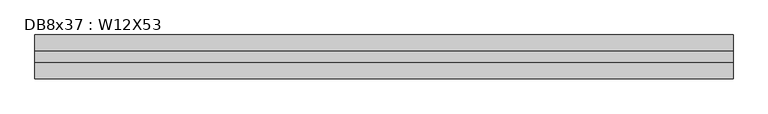
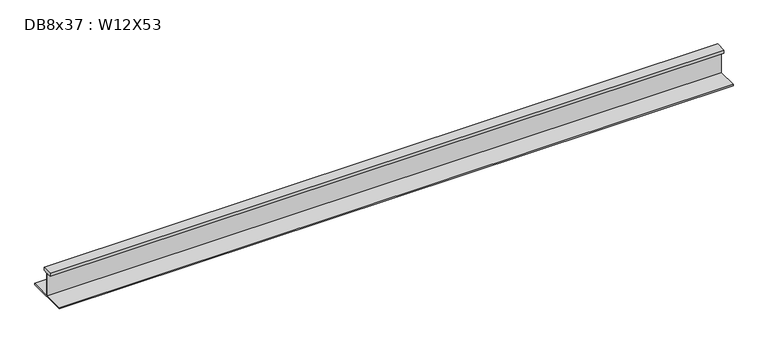
"""IFC4 building model written with IfcOpenShell, lengths in millimetres: beam geometry, DB8x37 : W12X53."""

from ifc_helpers import new_model, si_unit, frame, origin, place, context, project, spatial, polyline, outline, extrude, source, transform, mapped, element, save


def db8x37_w12x53_57ad42f3(model_context):
    return source(origin(), model_context, "Body", "SweptSolid", [
        extrude(outline(polyline([(38.1, 145.415), (38.1, 120.015), (2.921, 120.015), (2.921, -48.4505), (152.4, -48.4505), (152.4, -58.1025), (-152.4, -58.1025), (-152.4, -48.4505), (-2.921, -48.4505), (-2.921, 120.015), (-38.1, 120.015), (-38.1, 145.415), (38.1, 145.415)])), frame((-2497.8324214, 0.0, 0.0), z_axis=(1.0, 0.0, 0.0), x_axis=(0.0, 1.0, 0.0)), (0.0, 0.0, 1.0), 4871.291124),
    ])


if __name__ == "__main__":
    model = new_model("IFC4")
    model_context = context("Model", 3, world=origin())
    ifc_project = project(units=[si_unit("LENGTHUNIT", "METRE", prefix="MILLI")], contexts=[model_context])
    site = spatial("IfcSite", under=ifc_project)
    building = spatial("IfcBuilding", under=site)
    placement = place(None, origin())
    db8x37_w12x53_shape = db8x37_w12x53_57ad42f3(model_context)
    element("IfcBeam", 1, ObjectType="DB8x37 : W12X53", at=placement, inside=building, context=model_context, shape_type="MappedRepresentation", body=[
        mapped(db8x37_w12x53_shape, transform((0.0, 0.0, 0.0), x_axis=(1.0, 0.0, 0.0), y_axis=(0.0, 1.0, 0.0), z_axis=(0.0, 0.0, 1.0))),
    ])
    save(model, "model.ifc")

# Revit data of these elements
# Type "DB8x37 : W12X53"
#   Assembly Code = "B10"
#   W = 53
#   Length [instance default] = 5' - 0"
#   bf = 0' - 10"
#   d = 1' - 0.1"
#   k = 0' - 1 3/8"
#   k2 = 0' - 0.8"
#   tf = 0' - 0.575"
#   tw = 0' - 0.345"
#   A = 0.108333 SF
#   Structural Material [instance default] = Steel ASTM A992
# Element 1 (IfcBeam, "DB8x37 : W12X53")
#   Materials on its faces: "Steel ASTM A992"
# Materials
#   "Steel ASTM A992": class "Metal", colour RGB 199 199 199, transparency 0, Description = "Structural steel 50ksi", Cost = 0
